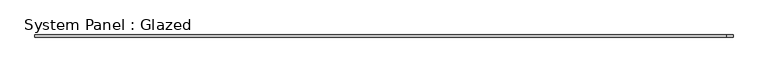
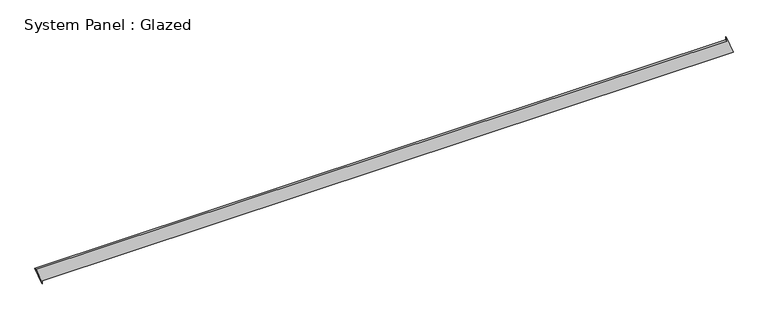
"""IFC4 building model written with IfcOpenShell, lengths in millimetres: plate geometry, System Panel : Glazed."""

import ifcopenshell
import ifcopenshell.guid

model = None  # the IFC model being written
_history = None  # IfcOwnerHistory: only IFC2X3 demands one
_inside = {}  # id of a spatial element -> (the spatial element, [elements in it])
_under = {}  # id of a project, library or spatial element -> (it, [spatial elements below it])
_declared = {}  # id of a project -> (the project, [libraries it declares])
_typed = {}  # id of a type object -> (the type object, [elements of that type])
_made_of = {}  # id of a material, layer set ... -> (it, [elements and type objects made of it])


def new_model(schema):
    """Start an empty IFC model of exactly this schema.

    Asked for "IFC4X3", IfcOpenShell would pick the latest addendum, in which some entities
    have other attributes; the version numbers below select the first issue.
    IFC2X3 requires an IfcOwnerHistory on every rooted entity: one is made here for all.
    """
    global model, _history
    if schema == "IFC4X3":
        model = ifcopenshell.file(schema_version=(4, 3, 0, 0))
    else:
        model = ifcopenshell.file(schema=schema)
    _inside.clear()
    _under.clear()
    _declared.clear()
    _typed.clear()
    _made_of.clear()
    _history = None
    if model.schema == "IFC2X3":
        org = make("IfcOrganization", Name="unknown")
        user = make(
            "IfcPersonAndOrganization",
            ThePerson=make("IfcPerson", FamilyName="unknown"),
            TheOrganization=org,
        )
        app = make(
            "IfcApplication",
            ApplicationDeveloper=org,
            Version="unknown",
            ApplicationFullName="unknown",
            ApplicationIdentifier="unknown",
        )
        _history = make(
            "IfcOwnerHistory",
            OwningUser=user,
            OwningApplication=app,
            ChangeAction="ADDED",
            CreationDate=0,
        )
    return model


def make(cls, **values):
    """One entity of the class cls with the attributes given. An attribute that is None is left unset."""
    return model.create_entity(
        cls, **{name: value for name, value in values.items() if value is not None}
    )


def rooted(cls, **values):
    """An entity with a GlobalId (a new one), such as an element, a storey or a relation."""
    return make(cls, GlobalId=ifcopenshell.guid.new(), OwnerHistory=_history, **values)


def si_unit(unit_type, name, prefix=None):
    """IfcSIUnit, for example si_unit("LENGTHUNIT", "METRE", prefix="MILLI")."""
    return make("IfcSIUnit", UnitType=unit_type, Prefix=prefix, Name=name)


def assignment(units):
    """IfcUnitAssignment: the units of a project."""
    return None if units is None else make("IfcUnitAssignment", Units=units)


def point(xyz):
    """IfcCartesianPoint."""
    return None if xyz is None else make("IfcCartesianPoint", Coordinates=xyz)


def direction(xyz):
    """IfcDirection."""
    return None if xyz is None else make("IfcDirection", DirectionRatios=xyz)


def frame(location, z_axis=None, x_axis=None):
    """IfcAxis2Placement3D, a coordinate frame: its origin and axes. An axis left out is left unset."""
    return make(
        "IfcAxis2Placement3D",
        Location=point(location),
        Axis=direction(z_axis),
        RefDirection=direction(x_axis),
    )


def origin():
    """The frame at (0, 0, 0) with its axes left unset."""
    return frame((0.0, 0.0, 0.0))


def place(relative_to, where):
    """IfcLocalPlacement: puts the frame where relative to a parent placement (None: the world)."""
    return make(
        "IfcLocalPlacement", PlacementRelTo=relative_to, RelativePlacement=where
    )


def context(
    kind, dimensions, precision=None, world=None, true_north=None, identifier=None
):
    """IfcGeometricRepresentationContext, for example the 3D "Model" context."""
    return make(
        "IfcGeometricRepresentationContext",
        ContextIdentifier=identifier,
        ContextType=kind,
        CoordinateSpaceDimension=dimensions,
        Precision=precision,
        WorldCoordinateSystem=world,
        TrueNorth=true_north,
    )


def project(units=None, contexts=None):
    """IfcProject with its units and contexts."""
    return rooted(
        "IfcProject",
        Name="project",
        RepresentationContexts=contexts,
        UnitsInContext=assignment(units),
    )


def spatial(cls, under=None, at=None, **own):
    """A site, building, storey or space (cls), placed at a placement, below another one or the project."""
    s = rooted(cls, ObjectPlacement=at, **own)
    if under is not None:
        _under.setdefault(under.id(), (under, []))[1].append(s)
    return s


def polyline(points):
    """IfcPolyline through the points."""
    return make("IfcPolyline", Points=[point(p) for p in points])


def outline(outer, holes=None, kind="AREA"):
    """IfcArbitraryClosedProfileDef: a profile drawn as a closed curve; with holes, ...WithVoids."""
    if holes is None:
        return make("IfcArbitraryClosedProfileDef", ProfileType=kind, OuterCurve=outer)
    return make(
        "IfcArbitraryProfileDefWithVoids",
        ProfileType=kind,
        OuterCurve=outer,
        InnerCurves=holes,
    )


def extrude(swept, where, along, depth):
    """IfcExtrudedAreaSolid: the profile swept, set in the frame where, extruded along a direction by depth."""
    return make(
        "IfcExtrudedAreaSolid",
        SweptArea=swept,
        Position=where,
        ExtrudedDirection=direction(along),
        Depth=depth,
    )


def shape(context_of_items, identifier, shape_type, items):
    """IfcShapeRepresentation: the items that make up one representation, for example the "Body"."""
    return make(
        "IfcShapeRepresentation",
        ContextOfItems=context_of_items,
        RepresentationIdentifier=identifier,
        RepresentationType=shape_type,
        Items=items,
    )


def source(mapping_origin, context_of_items, identifier, shape_type, items):
    """IfcRepresentationMap: a shape defined once, which mapped items show again and again."""
    return make(
        "IfcRepresentationMap",
        MappingOrigin=mapping_origin,
        MappedRepresentation=shape(context_of_items, identifier, shape_type, items),
    )


def transform(
    local_origin,
    x_axis=None,
    y_axis=None,
    z_axis=None,
    scale=None,
    scale2=None,
    scale3=None,
    uniform=True,
):
    """IfcCartesianTransformationOperator3D, or its non-uniform kind. x_axis, y_axis, z_axis: its Axis1, 2, 3."""
    if uniform:
        return make(
            "IfcCartesianTransformationOperator3D",
            Axis1=direction(x_axis),
            Axis2=direction(y_axis),
            LocalOrigin=point(local_origin),
            Scale=scale,
            Axis3=direction(z_axis),
        )
    return make(
        "IfcCartesianTransformationOperator3DnonUniform",
        Axis1=direction(x_axis),
        Axis2=direction(y_axis),
        LocalOrigin=point(local_origin),
        Scale=scale,
        Axis3=direction(z_axis),
        Scale2=scale2,
        Scale3=scale3,
    )


def mapped(mapping_source, mapping_target):
    """IfcMappedItem: shows the shape of a source again, moved by a transform."""
    return make(
        "IfcMappedItem", MappingSource=mapping_source, MappingTarget=mapping_target
    )


def made_of(thing, what):
    """Note that an element or type object is made of a material, layer set ...; save() writes the relation."""
    if what is not None:
        _made_of.setdefault(what.id(), (what, []))[1].append(thing)
    return thing


def element(
    cls,
    number,
    at=None,
    inside=None,
    cuts=None,
    type_object=None,
    material=None,
    context=None,
    identifier="Body",
    shape_type=None,
    held_by="IfcProductDefinitionShape",
    body=None,
    shapes=None,
    **own,
):
    """One element of the class cls, such as IfcWall. Its Tag is "e" and its number.

    at: its placement. inside: the storey or other place that contains it. cuts: it is an
    opening in that element (IfcRelVoidsElement). A single representation is given by context,
    identifier, shape_type and body (its items); several are given by shapes. held_by: the class
    of the entity that holds the representations. save() writes the other relations.
    """
    e = rooted(cls, Tag="e%d" % number, ObjectPlacement=at, **own)
    if body is not None:
        shapes = [shape(context, identifier, shape_type, body)]
    if shapes is not None:
        e.Representation = make(held_by, Representations=shapes)
    if inside is not None:
        _inside.setdefault(inside.id(), (inside, []))[1].append(e)
    if cuts is not None:
        rooted(
            "IfcRelVoidsElement", RelatingBuildingElement=cuts, RelatedOpeningElement=e
        )
    if type_object is not None:
        _typed.setdefault(type_object.id(), (type_object, []))[1].append(e)
    return made_of(e, material)


def aggregate(whole, parts):
    """IfcRelAggregates: a whole, such as a stair, and the parts it consists of."""
    return rooted("IfcRelAggregates", RelatingObject=whole, RelatedObjects=parts)


def save(model, path):
    """Write the relations noted so far, then the file.

    IfcRelAggregates (storeys below a building ...), IfcRelContainedInSpatialStructure (elements
    in a storey), IfcRelDefinesByType, IfcRelAssociatesMaterial and IfcRelDeclares: one each for
    every whole, place, type object, material and project.
    """
    for whole, parts in _under.values():
        aggregate(whole, parts)
    for where, things in _inside.values():
        rooted(
            "IfcRelContainedInSpatialStructure",
            RelatedElements=things,
            RelatingStructure=where,
        )
    for kind, things in _typed.values():
        rooted("IfcRelDefinesByType", RelatedObjects=things, RelatingType=kind)
    for what, things in _made_of.values():
        rooted("IfcRelAssociatesMaterial", RelatedObjects=things, RelatingMaterial=what)
    for by, libraries in _declared.values():
        rooted("IfcRelDeclares", RelatingContext=by, RelatedDefinitions=libraries)
    model.write(path)


def system_panel_glazed_383bb218(model_context):
    return source(origin(), model_context, "Body", "SweptSolid", [
        extrude(outline(polyline([(0.0, -3956.8326568), (35.3553391, -3956.8326568), (35.3553391, 4027.6791424), (234.6435672, 3956.3630659), (199.2882281, 3956.3621746), (199.4894988, -4027.6791424), (0.0, -3956.8326568)])), frame((0.0, -49.5, 0.0), z_axis=(0.0, 1.0, 0.0), x_axis=(0.0, 0.0, 1.0)), (0.0, 0.0, 1.0), 25.0),
    ])


if __name__ == "__main__":
    model = new_model("IFC4")
    model_context = context("Model", 3, world=origin())
    ifc_project = project(units=[si_unit("LENGTHUNIT", "METRE", prefix="MILLI")], contexts=[model_context])
    site = spatial("IfcSite", under=ifc_project)
    building = spatial("IfcBuilding", under=site)
    placement = place(None, origin())
    system_panel_glazed_shape = system_panel_glazed_383bb218(model_context)
    element("IfcPlate", 1, ObjectType="System Panel : Glazed", at=placement, inside=building, context=model_context, shape_type="MappedRepresentation", body=[
        mapped(system_panel_glazed_shape, transform((0.0, 0.0, 0.0), x_axis=(1.0, 0.0, 0.0), y_axis=(0.0, 1.0, 0.0), z_axis=(0.0, 0.0, 1.0))),
    ])
    save(model, "model.ifc")

# Revit data of these elements
# Element 1 (IfcPlate, "System Panel : Glazed")
#   Materials on its faces: "Glass"
# Materials
#   "Glass": class "Glass", colour RGB 218 227 224, transparency 0.85, Description = "Soda Lime Glass", Cost = 0
